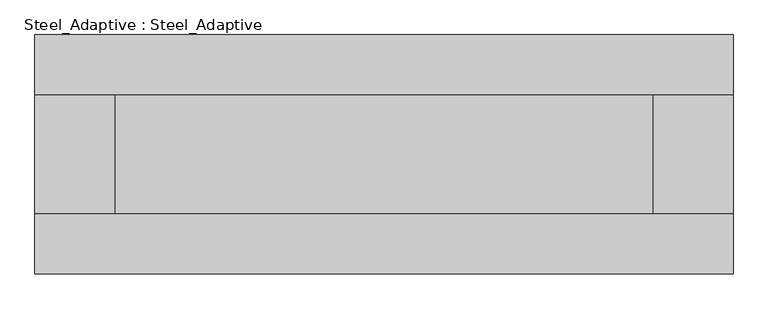
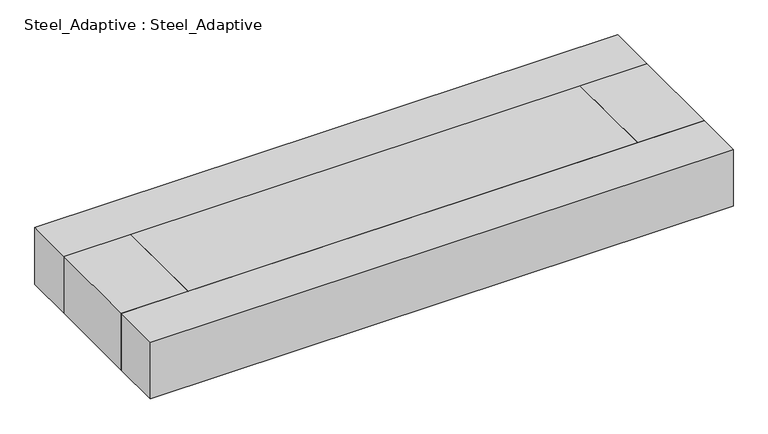
"""IFC4 building model written with IfcOpenShell, lengths in millimetres: proxy geometry, Steel_Adaptive : Steel_Adaptive."""

from ifc_helpers import new_model, si_unit, frame, origin, place, context, project, spatial, polyline, outline, extrude, source, transform, mapped, element, save


def steel_adaptive_steel_adaptive_233fae97(model_context):
    return source(origin(), model_context, "Body", "SweptSolid", [
        extrude(outline(polyline([(8750.0, 1500.0), (-8750.0, 1500.0), (-8750.0, 3000.0), (8750.0, 3000.0), (8750.0, 1500.0)])), frame((0.0, 0.0, 130700.0), z_axis=(0.0, 0.0, 1.0), x_axis=(1.0, 0.0, 0.0)), (0.0, 0.0, 1.0), 1800.0),
        extrude(outline(polyline([(-8750.0, -1500.0), (8750.0, -1500.0), (8750.0, -3000.0), (-8750.0, -3000.0), (-8750.0, -1500.0)])), frame((0.0, 0.0, 130700.0), z_axis=(0.0, 0.0, 1.0), x_axis=(1.0, 0.0, 0.0)), (0.0, 0.0, 1.0), 1800.0),
        extrude(outline(polyline([(6750.0, -1500.0), (6750.0, 1500.0), (8750.0, 1500.0), (8750.0, -1500.0), (6750.0, -1500.0)])), frame((0.0, 0.0, 130700.0), z_axis=(0.0, 0.0, 1.0), x_axis=(1.0, 0.0, 0.0)), (0.0, 0.0, 1.0), 1800.0),
        extrude(outline(polyline([(-6750.0, 1500.0), (-6750.0, -1500.0), (-8750.0, -1500.0), (-8750.0, 1500.0), (-6750.0, 1500.0)])), frame((0.0, 0.0, 130700.0), z_axis=(0.0, 0.0, 1.0), x_axis=(1.0, 0.0, 0.0)), (0.0, 0.0, 1.0), 1800.0),
        extrude(outline(polyline([(-6750.0, -1500.0), (-6750.0, 1500.0), (6750.0, 1500.0), (6750.0, -1500.0), (-6750.0, -1500.0)])), frame((0.0, 0.0, 130700.0), z_axis=(0.0, 0.0, 1.0), x_axis=(1.0, 0.0, 0.0)), (0.0, 0.0, 1.0), 1800.0),
    ])


if __name__ == "__main__":
    model = new_model("IFC4")
    model_context = context("Model", 3, world=origin())
    ifc_project = project(units=[si_unit("LENGTHUNIT", "METRE", prefix="MILLI")], contexts=[model_context])
    site = spatial("IfcSite", under=ifc_project)
    building = spatial("IfcBuilding", under=site)
    placement = place(None, origin())
    steel_adaptive_steel_adaptive_shape = steel_adaptive_steel_adaptive_233fae97(model_context)
    element("IfcBuildingElementProxy", 1, Name="Steel_Adaptive : Steel_Adaptive", ObjectType="Steel_Adaptive : Steel_Adaptive", at=placement, inside=building, context=model_context, shape_type="MappedRepresentation", body=[
        mapped(steel_adaptive_steel_adaptive_shape, transform((0.0, 0.0, 0.0), x_axis=(1.0, 0.0, 0.0), y_axis=(0.0, 1.0, 0.0), z_axis=(0.0, 0.0, 1.0))),
    ])
    save(model, "model.ifc")

# Revit data of these elements
# Type "Steel_Adaptive : Steel_Adaptive"
#   Width = 3000 mm
#   Top Width = 3000 mm
#   Length = 21000 mm
#   Height [instance default] = 80000 mm
#   Default Elevation = 0
# Element 1 (IfcBuildingElementProxy, "Steel_Adaptive : Steel_Adaptive")
#   Height = 130700 mm
